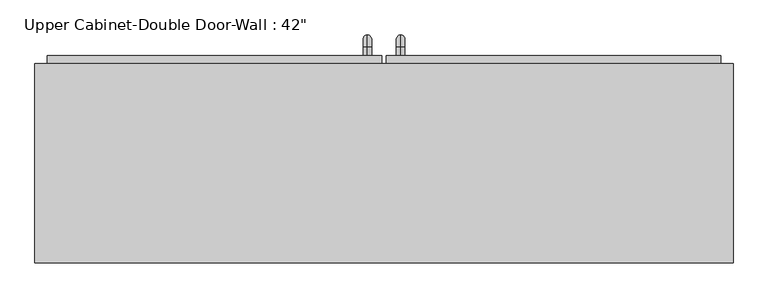
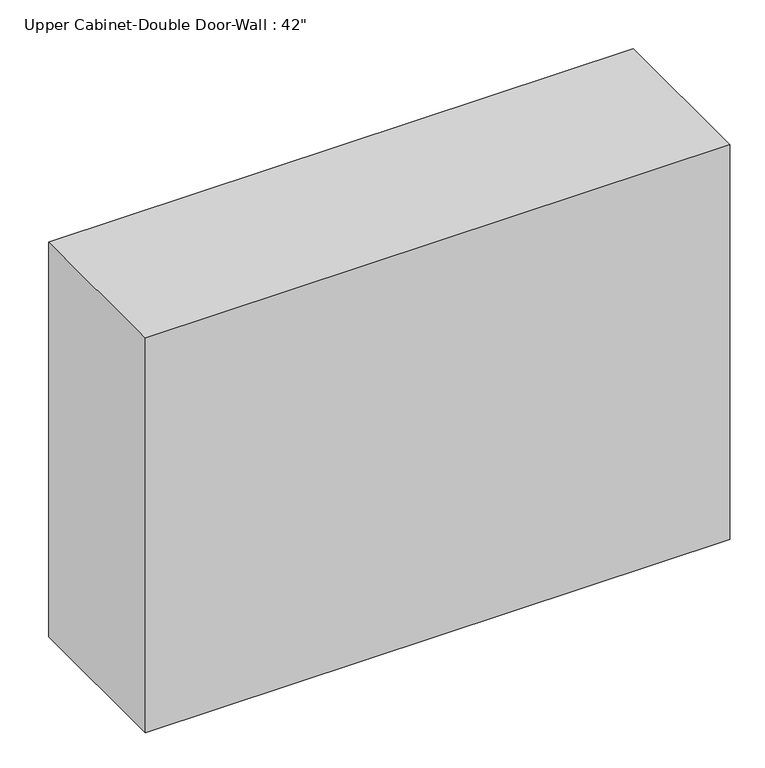
"""IFC4 building model written with IfcOpenShell, lengths in millimetres: furniture geometry."""

import ifcopenshell
import ifcopenshell.guid

model = None  # the IFC model being written
_history = None  # IfcOwnerHistory: only IFC2X3 demands one
_inside = {}  # id of a spatial element -> (the spatial element, [elements in it])
_under = {}  # id of a project, library or spatial element -> (it, [spatial elements below it])
_declared = {}  # id of a project -> (the project, [libraries it declares])
_typed = {}  # id of a type object -> (the type object, [elements of that type])
_made_of = {}  # id of a material, layer set ... -> (it, [elements and type objects made of it])


def new_model(schema):
    """Start an empty IFC model of exactly this schema.

    Asked for "IFC4X3", IfcOpenShell would pick the latest addendum, in which some entities
    have other attributes; the version numbers below select the first issue.
    IFC2X3 requires an IfcOwnerHistory on every rooted entity: one is made here for all.
    """
    global model, _history
    if schema == "IFC4X3":
        model = ifcopenshell.file(schema_version=(4, 3, 0, 0))
    else:
        model = ifcopenshell.file(schema=schema)
    _inside.clear()
    _under.clear()
    _declared.clear()
    _typed.clear()
    _made_of.clear()
    _history = None
    if model.schema == "IFC2X3":
        org = make("IfcOrganization", Name="unknown")
        user = make(
            "IfcPersonAndOrganization",
            ThePerson=make("IfcPerson", FamilyName="unknown"),
            TheOrganization=org,
        )
        app = make(
            "IfcApplication",
            ApplicationDeveloper=org,
            Version="unknown",
            ApplicationFullName="unknown",
            ApplicationIdentifier="unknown",
        )
        _history = make(
            "IfcOwnerHistory",
            OwningUser=user,
            OwningApplication=app,
            ChangeAction="ADDED",
            CreationDate=0,
        )
    return model


def make(cls, **values):
    """One entity of the class cls with the attributes given. An attribute that is None is left unset."""
    return model.create_entity(
        cls, **{name: value for name, value in values.items() if value is not None}
    )


def rooted(cls, **values):
    """An entity with a GlobalId (a new one), such as an element, a storey or a relation."""
    return make(cls, GlobalId=ifcopenshell.guid.new(), OwnerHistory=_history, **values)


def si_unit(unit_type, name, prefix=None):
    """IfcSIUnit, for example si_unit("LENGTHUNIT", "METRE", prefix="MILLI")."""
    return make("IfcSIUnit", UnitType=unit_type, Prefix=prefix, Name=name)


def assignment(units):
    """IfcUnitAssignment: the units of a project."""
    return None if units is None else make("IfcUnitAssignment", Units=units)


def point(xyz):
    """IfcCartesianPoint."""
    return None if xyz is None else make("IfcCartesianPoint", Coordinates=xyz)


def direction(xyz):
    """IfcDirection."""
    return None if xyz is None else make("IfcDirection", DirectionRatios=xyz)


def frame(location, z_axis=None, x_axis=None):
    """IfcAxis2Placement3D, a coordinate frame: its origin and axes. An axis left out is left unset."""
    return make(
        "IfcAxis2Placement3D",
        Location=point(location),
        Axis=direction(z_axis),
        RefDirection=direction(x_axis),
    )


def origin():
    """The frame at (0, 0, 0) with its axes left unset."""
    return frame((0.0, 0.0, 0.0))


def place(relative_to, where):
    """IfcLocalPlacement: puts the frame where relative to a parent placement (None: the world)."""
    return make(
        "IfcLocalPlacement", PlacementRelTo=relative_to, RelativePlacement=where
    )


def context(
    kind, dimensions, precision=None, world=None, true_north=None, identifier=None
):
    """IfcGeometricRepresentationContext, for example the 3D "Model" context."""
    return make(
        "IfcGeometricRepresentationContext",
        ContextIdentifier=identifier,
        ContextType=kind,
        CoordinateSpaceDimension=dimensions,
        Precision=precision,
        WorldCoordinateSystem=world,
        TrueNorth=true_north,
    )


def project(units=None, contexts=None):
    """IfcProject with its units and contexts."""
    return rooted(
        "IfcProject",
        Name="project",
        RepresentationContexts=contexts,
        UnitsInContext=assignment(units),
    )


def spatial(cls, under=None, at=None, **own):
    """A site, building, storey or space (cls), placed at a placement, below another one or the project."""
    s = rooted(cls, ObjectPlacement=at, **own)
    if under is not None:
        _under.setdefault(under.id(), (under, []))[1].append(s)
    return s


def polyline(points):
    """IfcPolyline through the points."""
    return make("IfcPolyline", Points=[point(p) for p in points])


def circle_curve(where, radius):
    """IfcCircle in the frame where."""
    return make("IfcCircle", Position=where, Radius=radius)


def ellipse_curve(where, semi_axis1, semi_axis2):
    """IfcEllipse in the frame where."""
    return make(
        "IfcEllipse", Position=where, SemiAxis1=semi_axis1, SemiAxis2=semi_axis2
    )


def trimmed(basis, trim1, trim2, sense, master):
    """IfcTrimmedCurve: the piece of a basis curve between two trims."""
    return make(
        "IfcTrimmedCurve",
        BasisCurve=basis,
        Trim1=trim1,
        Trim2=trim2,
        SenseAgreement=sense,
        MasterRepresentation=master,
    )


def outline(outer, holes=None, kind="AREA"):
    """IfcArbitraryClosedProfileDef: a profile drawn as a closed curve; with holes, ...WithVoids."""
    if holes is None:
        return make("IfcArbitraryClosedProfileDef", ProfileType=kind, OuterCurve=outer)
    return make(
        "IfcArbitraryProfileDefWithVoids",
        ProfileType=kind,
        OuterCurve=outer,
        InnerCurves=holes,
    )


def extrude(swept, where, along, depth):
    """IfcExtrudedAreaSolid: the profile swept, set in the frame where, extruded along a direction by depth."""
    return make(
        "IfcExtrudedAreaSolid",
        SweptArea=swept,
        Position=where,
        ExtrudedDirection=direction(along),
        Depth=depth,
    )


def faces_of(points, faces, orient=None, outer=None):
    """IfcFace entities. A face is a list of loops; a loop is a list of indices into points, from 0.

    orient and outer hold one flag for each loop. By default every Orientation is true, the
    first loop of a face is its IfcFaceOuterBound and the others are IfcFaceBound.
    """
    made = []
    for i, loops in enumerate(faces):
        bounds = []
        for j, loop in enumerate(loops):
            is_outer = j == 0 if outer is None else outer[i][j]
            bounds.append(
                make(
                    "IfcFaceOuterBound" if is_outer else "IfcFaceBound",
                    Bound=make("IfcPolyLoop", Polygon=[points[k] for k in loop]),
                    Orientation=True if orient is None else orient[i][j],
                )
            )
        made.append(make("IfcFace", Bounds=bounds))
    return made


def faceted_brep(points, faces, orient=None, outer=None, voids=None):
    """IfcFacetedBrep: a solid bounded by flat faces; with voids (closed shells), ...WithVoids."""
    shared = [point(p) for p in points]
    hull = make("IfcClosedShell", CfsFaces=faces_of(shared, faces, orient, outer))
    if voids is None:
        return make("IfcFacetedBrep", Outer=hull)
    return make(
        "IfcFacetedBrepWithVoids",
        Outer=hull,
        Voids=[
            make(cls, CfsFaces=faces_of(shared, fs, o, b)) for cls, fs, o, b in voids
        ],
    )


def shape(context_of_items, identifier, shape_type, items):
    """IfcShapeRepresentation: the items that make up one representation, for example the "Body"."""
    return make(
        "IfcShapeRepresentation",
        ContextOfItems=context_of_items,
        RepresentationIdentifier=identifier,
        RepresentationType=shape_type,
        Items=items,
    )


def source(mapping_origin, context_of_items, identifier, shape_type, items):
    """IfcRepresentationMap: a shape defined once, which mapped items show again and again."""
    return make(
        "IfcRepresentationMap",
        MappingOrigin=mapping_origin,
        MappedRepresentation=shape(context_of_items, identifier, shape_type, items),
    )


def transform(
    local_origin,
    x_axis=None,
    y_axis=None,
    z_axis=None,
    scale=None,
    scale2=None,
    scale3=None,
    uniform=True,
):
    """IfcCartesianTransformationOperator3D, or its non-uniform kind. x_axis, y_axis, z_axis: its Axis1, 2, 3."""
    if uniform:
        return make(
            "IfcCartesianTransformationOperator3D",
            Axis1=direction(x_axis),
            Axis2=direction(y_axis),
            LocalOrigin=point(local_origin),
            Scale=scale,
            Axis3=direction(z_axis),
        )
    return make(
        "IfcCartesianTransformationOperator3DnonUniform",
        Axis1=direction(x_axis),
        Axis2=direction(y_axis),
        LocalOrigin=point(local_origin),
        Scale=scale,
        Axis3=direction(z_axis),
        Scale2=scale2,
        Scale3=scale3,
    )


def mapped(mapping_source, mapping_target):
    """IfcMappedItem: shows the shape of a source again, moved by a transform."""
    return make(
        "IfcMappedItem", MappingSource=mapping_source, MappingTarget=mapping_target
    )


def made_of(thing, what):
    """Note that an element or type object is made of a material, layer set ...; save() writes the relation."""
    if what is not None:
        _made_of.setdefault(what.id(), (what, []))[1].append(thing)
    return thing


def element(
    cls,
    number,
    at=None,
    inside=None,
    cuts=None,
    type_object=None,
    material=None,
    context=None,
    identifier="Body",
    shape_type=None,
    held_by="IfcProductDefinitionShape",
    body=None,
    shapes=None,
    **own,
):
    """One element of the class cls, such as IfcWall. Its Tag is "e" and its number.

    at: its placement. inside: the storey or other place that contains it. cuts: it is an
    opening in that element (IfcRelVoidsElement). A single representation is given by context,
    identifier, shape_type and body (its items); several are given by shapes. held_by: the class
    of the entity that holds the representations. save() writes the other relations.
    """
    e = rooted(cls, Tag="e%d" % number, ObjectPlacement=at, **own)
    if body is not None:
        shapes = [shape(context, identifier, shape_type, body)]
    if shapes is not None:
        e.Representation = make(held_by, Representations=shapes)
    if inside is not None:
        _inside.setdefault(inside.id(), (inside, []))[1].append(e)
    if cuts is not None:
        rooted(
            "IfcRelVoidsElement", RelatingBuildingElement=cuts, RelatedOpeningElement=e
        )
    if type_object is not None:
        _typed.setdefault(type_object.id(), (type_object, []))[1].append(e)
    return made_of(e, material)


def aggregate(whole, parts):
    """IfcRelAggregates: a whole, such as a stair, and the parts it consists of."""
    return rooted("IfcRelAggregates", RelatingObject=whole, RelatedObjects=parts)


def save(model, path):
    """Write the relations noted so far, then the file.

    IfcRelAggregates (storeys below a building ...), IfcRelContainedInSpatialStructure (elements
    in a storey), IfcRelDefinesByType, IfcRelAssociatesMaterial and IfcRelDeclares: one each for
    every whole, place, type object, material and project.
    """
    for whole, parts in _under.values():
        aggregate(whole, parts)
    for where, things in _inside.values():
        rooted(
            "IfcRelContainedInSpatialStructure",
            RelatedElements=things,
            RelatingStructure=where,
        )
    for kind, things in _typed.values():
        rooted("IfcRelDefinesByType", RelatedObjects=things, RelatingType=kind)
    for what, things in _made_of.values():
        rooted("IfcRelAssociatesMaterial", RelatedObjects=things, RelatingMaterial=what)
    for by, libraries in _declared.values():
        rooted("IfcRelDeclares", RelatingContext=by, RelatedDefinitions=libraries)
    model.write(path)


def plane_surface(at):
    """IfcPlane: the flat surface through the origin of the frame at, square to its z axis."""
    return make("IfcPlane", Position=at)


def cylinder_surface(at, radius):
    """IfcCylindricalSurface: all points at the distance radius from the z axis of the frame at."""
    return make("IfcCylindricalSurface", Position=at, Radius=radius)


def revolved_surface(curve, axis_point, axis_direction):
    """IfcSurfaceOfRevolution: the curve turned about the line through axis_point along axis_direction."""
    return make(
        "IfcSurfaceOfRevolution",
        SweptCurve=make("IfcArbitraryOpenProfileDef", ProfileType="CURVE", Curve=curve),
        AxisPosition=make("IfcAxis1Placement", Location=point(axis_point), Axis=direction(axis_direction)),
    )


def advanced_brep(points, edges, surfaces, faces):
    """IfcAdvancedBrep: a solid bounded by faces that lie on surfaces and meet in shared edges.

    An edge is (start, end): straight between two places in points (the first is 0);
    or (start, end, curve); or (start, end, curve, False) where it runs against its curve.
    A face is (place in surfaces, loops), or (place, loops, False) where it looks against
    its surface's normal. A loop lists edges by number (the first is 1), with a minus sign
    where the edge is run from its end to its start. The first loop is the outer one.
    """
    corners = [point(p) for p in points]
    vertices = [make("IfcVertexPoint", VertexGeometry=c) for c in corners]
    made = []
    for start, end, *more in edges:
        made.append(
            make(
                "IfcEdgeCurve",
                EdgeStart=vertices[start],
                EdgeEnd=vertices[end],
                EdgeGeometry=more[0] if more else make("IfcPolyline", Points=[corners[start], corners[end]]),
                SameSense=more[1] if len(more) > 1 else True,
            )
        )
    hull = []
    for where, loops, *sense in faces:
        bounds = []
        for j, loop in enumerate(loops):
            ring = [make("IfcOrientedEdge", EdgeElement=made[abs(k) - 1], Orientation=k > 0) for k in loop]
            bounds.append(
                make(
                    "IfcFaceOuterBound" if j == 0 else "IfcFaceBound",
                    Bound=make("IfcEdgeLoop", EdgeList=ring),
                    Orientation=True,
                )
            )
        hull.append(make("IfcAdvancedFace", Bounds=bounds, FaceSurface=surfaces[where], SameSense=sense[0] if sense else True))
    return make("IfcAdvancedBrep", Outer=make("IfcClosedShell", CfsFaces=hull))


def furniture_35403546(model_context):
    return source(origin(), model_context, "Body", "SolidModel", [
        faceted_brep([(-503.6288372, 61.9125, 2133.6), (-503.6288372, 61.9125, 1371.6), (563.1711628, 61.9125, 1371.6), (563.1711628, 61.9125, 2133.6), (-503.6288372, 366.7125, 2133.6), (563.1711628, 366.7125, 2133.6), (563.1711628, 366.7125, 1371.6), (-503.6288372, 366.7125, 1371.6), (-484.5788372, 366.7125, 2114.55), (-484.5788372, 366.7125, 1390.65), (544.1211628, 366.7125, 1390.65), (544.1211628, 366.7125, 2114.55), (544.1211628, 80.9625, 2114.55), (-484.5788372, 80.9625, 2114.55), (544.1211628, 80.9625, 1390.65), (-484.5788372, 80.9625, 1390.65)], [[[0, 1, 2, 3]], [[4, 5, 6, 7], [8, 9, 10, 11]], [[1, 0, 4, 7]], [[2, 1, 7, 6]], [[3, 2, 6, 5]], [[0, 3, 5, 4]], [[8, 11, 12, 13]], [[11, 10, 14, 12]], [[10, 9, 15, 14]], [[9, 8, 13, 15]], [[13, 12, 14, 15]]]),
        advanced_brep(
        [(55.1711628, 379.4125, 1517.65), (55.1711628, 379.4125, 1530.35), (55.1711628, 392.1125, 1517.65), (55.1711628, 392.1125, 1530.35), (55.1711628, 411.1625, 1511.3), (55.1711628, 398.4625, 1511.3), (55.1711628, 398.4625, 1435.1), (55.1711628, 411.1625, 1435.1), (55.1711628, 392.1125, 1416.05), (55.1711628, 392.1125, 1428.75), (55.1711628, 379.4125, 1428.75), (55.1711628, 379.4125, 1416.05)],
        [
            (0, 1, circle_curve(frame((55.1711628, 379.4125, 1524.0), z_axis=(0.0, -1.0, 0.0), x_axis=(0.0, 0.0, -1.0)), 6.35)),
            (1, 0, circle_curve(frame((55.1711628, 379.4125, 1524.0), z_axis=(0.0, -1.0, 0.0), x_axis=(0.0, 0.0, -1.0)), 6.35)),
            (0, 2),
            (2, 3, circle_curve(frame((55.1711628, 392.1125, 1524.0), z_axis=(0.0, -1.0, 0.0), x_axis=(0.0, 0.0, -1.0)), 6.35)),
            (3, 1),
            (3, 2, circle_curve(frame((55.1711628, 392.1125, 1524.0), z_axis=(0.0, -1.0, 0.0), x_axis=(0.0, 0.0, -1.0)), 6.35)),
            (4, 3, circle_curve(frame((55.1711628, 392.1125, 1511.3), z_axis=(1.0, 0.0, 0.0), x_axis=(0.0, 0.0, 1.0)), 19.05)),
            (2, 5, circle_curve(frame((55.1711628, 392.1125, 1511.3), z_axis=(-1.0, 0.0, 0.0), x_axis=(0.0, 0.0, 1.0)), 6.35)),
            (5, 4, circle_curve(frame((55.1711628, 404.8125, 1511.3), z_axis=(0.0, 0.0, 1.0), x_axis=(0.0, -1.0, 0.0)), 6.35)),
            (4, 5, circle_curve(frame((55.1711628, 404.8125, 1511.3), z_axis=(0.0, 0.0, 1.0), x_axis=(0.0, -1.0, 0.0)), 6.35)),
            (5, 6),
            (6, 7, circle_curve(frame((55.1711628, 404.8125, 1435.1), z_axis=(0.0, 0.0, 1.0), x_axis=(0.0, -1.0, 0.0)), 6.35)),
            (7, 4),
            (7, 6, circle_curve(frame((55.1711628, 404.8125, 1435.1), z_axis=(0.0, 0.0, 1.0), x_axis=(0.0, -1.0, 0.0)), 6.35)),
            (8, 7, circle_curve(frame((55.1711628, 392.1125, 1435.1), z_axis=(1.0, 0.0, 0.0), x_axis=(0.0, 1.0, 0.0)), 19.05)),
            (6, 9, circle_curve(frame((55.1711628, 392.1125, 1435.1), z_axis=(-1.0, 0.0, 0.0), x_axis=(0.0, 1.0, 0.0)), 6.35)),
            (9, 8, circle_curve(frame((55.1711628, 392.1125, 1422.4), z_axis=(0.0, 1.0, 0.0), x_axis=(0.0, 0.0, 1.0)), 6.35)),
            (8, 9, circle_curve(frame((55.1711628, 392.1125, 1422.4), z_axis=(0.0, 1.0, 0.0), x_axis=(0.0, 0.0, 1.0)), 6.35)),
            (10, 11, circle_curve(frame((55.1711628, 379.4125, 1422.4), z_axis=(0.0, -1.0, 0.0), x_axis=(0.0, 0.0, 1.0)), 6.35)),
            (11, 10, circle_curve(frame((55.1711628, 379.4125, 1422.4), z_axis=(0.0, -1.0, 0.0), x_axis=(0.0, 0.0, 1.0)), 6.35)),
            (9, 10),
            (11, 8),
        ],
        [
            plane_surface(frame((48.8211628, 379.4125, 1524.0), z_axis=(0.0, -1.0, 0.0), x_axis=(0.0, 0.0, 1.0))),
            cylinder_surface(frame((55.1711628, 379.4125, 1524.0), z_axis=(0.0, -1.0, 0.0), x_axis=(0.0, 0.0, -1.0)), 6.35),
            revolved_surface(trimmed(ellipse_curve(frame((55.1711628, 392.1125, 1524.0), z_axis=(0.0, -1.0, 0.0), x_axis=(0.0, 0.0, -1.0)), 6.35, 6.35), [point((55.1711628, 392.1125, 1517.65))], [point((55.1711628, 392.1125, 1530.35))], True, "CARTESIAN"), (55.1711628, 392.1125, 1511.3), (-1.0, 0.0, 0.0)),
            revolved_surface(trimmed(ellipse_curve(frame((55.1711628, 392.1125, 1524.0), z_axis=(0.0, -1.0, 0.0), x_axis=(0.0, 0.0, -1.0)), 6.35, 6.35), [point((55.1711628, 392.1125, 1530.35))], [point((55.1711628, 392.1125, 1517.65))], True, "CARTESIAN"), (55.1711628, 392.1125, 1511.3), (-1.0, 0.0, 0.0)),
            cylinder_surface(frame((55.1711628, 404.8125, 1511.3), z_axis=(0.0, 0.0, 1.0), x_axis=(0.0, -1.0, 0.0)), 6.35),
            revolved_surface(trimmed(ellipse_curve(frame((55.1711628, 404.8125, 1435.1), z_axis=(0.0, 0.0, 1.0), x_axis=(0.0, -1.0, 0.0)), 6.35, 6.35), [point((55.1711628, 398.4625, 1435.1))], [point((55.1711628, 411.1625, 1435.1))], True, "CARTESIAN"), (55.1711628, 392.1125, 1435.1), (-1.0, 0.0, 0.0)),
            revolved_surface(trimmed(ellipse_curve(frame((55.1711628, 404.8125, 1435.1), z_axis=(0.0, 0.0, 1.0), x_axis=(0.0, -1.0, 0.0)), 6.35, 6.35), [point((55.1711628, 411.1625, 1435.1))], [point((55.1711628, 398.4625, 1435.1))], True, "CARTESIAN"), (55.1711628, 392.1125, 1435.1), (-1.0, 0.0, 0.0)),
            plane_surface(frame((48.8211628, 379.4125, 1422.4), z_axis=(0.0, -1.0, 0.0), x_axis=(0.0, 0.0, -1.0))),
            cylinder_surface(frame((55.1711628, 392.1125, 1422.4), z_axis=(0.0, 1.0, 0.0), x_axis=(0.0, 0.0, 1.0)), 6.35),
        ],
        [
            (0, [[1, 2]]),
            (1, [[-1, 3, 4, 5]]),
            (1, [[-2, -5, 6, -3]]),
            (2, [[7, -4, 8, 9]]),
            (3, [[-8, -6, -7, 10]]),
            (4, [[-9, 11, 12, 13]]),
            (4, [[-10, -13, 14, -11]]),
            (5, [[15, -12, 16, 17]]),
            (6, [[-16, -14, -15, 18]]),
            (7, [[19, 20]]),
            (8, [[-17, 21, -20, 22]]),
            (8, [[-18, -22, -19, -21]]),
        ],
    ),
        advanced_brep(
        [(4.3711628, 379.4125, 1517.65), (4.3711628, 379.4125, 1530.35), (4.3711628, 392.1125, 1517.65), (4.3711628, 392.1125, 1530.35), (4.3711628, 411.1625, 1511.3), (4.3711628, 398.4625, 1511.3), (4.3711628, 398.4625, 1435.1), (4.3711628, 411.1625, 1435.1), (4.3711628, 392.1125, 1416.05), (4.3711628, 392.1125, 1428.75), (4.3711628, 379.4125, 1428.75), (4.3711628, 379.4125, 1416.05)],
        [
            (0, 1, circle_curve(frame((4.3711628, 379.4125, 1524.0), z_axis=(0.0, -1.0, 0.0), x_axis=(0.0, 0.0, 1.0)), 6.35)),
            (1, 0, circle_curve(frame((4.3711628, 379.4125, 1524.0), z_axis=(0.0, -1.0, 0.0), x_axis=(0.0, 0.0, 1.0)), 6.35)),
            (0, 2),
            (2, 3, circle_curve(frame((4.3711628, 392.1125, 1524.0), z_axis=(0.0, -1.0, 0.0), x_axis=(0.0, 0.0, 1.0)), 6.35)),
            (3, 1),
            (3, 2, circle_curve(frame((4.3711628, 392.1125, 1524.0), z_axis=(0.0, -1.0, 0.0), x_axis=(0.0, 0.0, 1.0)), 6.35)),
            (4, 3, circle_curve(frame((4.3711628, 392.1125, 1511.3), z_axis=(1.0, 0.0, 0.0), x_axis=(0.0, 0.0, 1.0)), 19.05)),
            (2, 5, circle_curve(frame((4.3711628, 392.1125, 1511.3), z_axis=(-1.0, 0.0, 0.0), x_axis=(0.0, 0.0, 1.0)), 6.35)),
            (5, 4, circle_curve(frame((4.3711628, 404.8125, 1511.3), z_axis=(0.0, 0.0, 1.0), x_axis=(0.0, 1.0, 0.0)), 6.35)),
            (4, 5, circle_curve(frame((4.3711628, 404.8125, 1511.3), z_axis=(0.0, 0.0, 1.0), x_axis=(0.0, 1.0, 0.0)), 6.35)),
            (5, 6),
            (6, 7, circle_curve(frame((4.3711628, 404.8125, 1435.1), z_axis=(0.0, 0.0, 1.0), x_axis=(0.0, 1.0, 0.0)), 6.35)),
            (7, 4),
            (7, 6, circle_curve(frame((4.3711628, 404.8125, 1435.1), z_axis=(0.0, 0.0, 1.0), x_axis=(0.0, 1.0, 0.0)), 6.35)),
            (8, 7, circle_curve(frame((4.3711628, 392.1125, 1435.1), z_axis=(1.0, 0.0, 0.0), x_axis=(0.0, 1.0, 0.0)), 19.05)),
            (6, 9, circle_curve(frame((4.3711628, 392.1125, 1435.1), z_axis=(-1.0, 0.0, 0.0), x_axis=(0.0, 1.0, 0.0)), 6.35)),
            (9, 8, circle_curve(frame((4.3711628, 392.1125, 1422.4), z_axis=(0.0, 1.0, 0.0), x_axis=(0.0, 0.0, -1.0)), 6.35)),
            (8, 9, circle_curve(frame((4.3711628, 392.1125, 1422.4), z_axis=(0.0, 1.0, 0.0), x_axis=(0.0, 0.0, -1.0)), 6.35)),
            (10, 11, circle_curve(frame((4.3711628, 379.4125, 1422.4), z_axis=(0.0, -1.0, 0.0), x_axis=(0.0, 0.0, -1.0)), 6.35)),
            (11, 10, circle_curve(frame((4.3711628, 379.4125, 1422.4), z_axis=(0.0, -1.0, 0.0), x_axis=(0.0, 0.0, -1.0)), 6.35)),
            (9, 10),
            (11, 8),
        ],
        [
            plane_surface(frame((-1.9788372, 379.4125, 1524.0), z_axis=(0.0, -1.0, 0.0), x_axis=(0.0, 0.0, 1.0))),
            cylinder_surface(frame((4.3711628, 379.4125, 1524.0), z_axis=(0.0, -1.0, 0.0), x_axis=(0.0, 0.0, 1.0)), 6.35),
            revolved_surface(trimmed(ellipse_curve(frame((4.3711628, 392.1125, 1524.0), z_axis=(0.0, -1.0, 0.0), x_axis=(0.0, 0.0, 1.0)), 6.35, 6.35), [point((4.3711628, 392.1125, 1517.65))], [point((4.3711628, 392.1125, 1530.35))], True, "CARTESIAN"), (4.3711628, 392.1125, 1511.3), (-1.0, 0.0, 0.0)),
            revolved_surface(trimmed(ellipse_curve(frame((4.3711628, 392.1125, 1524.0), z_axis=(0.0, -1.0, 0.0), x_axis=(0.0, 0.0, 1.0)), 6.35, 6.35), [point((4.3711628, 392.1125, 1530.35))], [point((4.3711628, 392.1125, 1517.65))], True, "CARTESIAN"), (4.3711628, 392.1125, 1511.3), (-1.0, 0.0, 0.0)),
            cylinder_surface(frame((4.3711628, 404.8125, 1511.3), z_axis=(0.0, 0.0, 1.0), x_axis=(0.0, 1.0, 0.0)), 6.35),
            revolved_surface(trimmed(ellipse_curve(frame((4.3711628, 404.8125, 1435.1), z_axis=(0.0, 0.0, 1.0), x_axis=(0.0, 1.0, 0.0)), 6.35, 6.35), [point((4.3711628, 398.4625, 1435.1))], [point((4.3711628, 411.1625, 1435.1))], True, "CARTESIAN"), (4.3711628, 392.1125, 1435.1), (-1.0, 0.0, 0.0)),
            revolved_surface(trimmed(ellipse_curve(frame((4.3711628, 404.8125, 1435.1), z_axis=(0.0, 0.0, 1.0), x_axis=(0.0, 1.0, 0.0)), 6.35, 6.35), [point((4.3711628, 411.1625, 1435.1))], [point((4.3711628, 398.4625, 1435.1))], True, "CARTESIAN"), (4.3711628, 392.1125, 1435.1), (-1.0, 0.0, 0.0)),
            plane_surface(frame((-1.9788372, 379.4125, 1422.4), z_axis=(0.0, -1.0, 0.0), x_axis=(0.0, 0.0, -1.0))),
            cylinder_surface(frame((4.3711628, 392.1125, 1422.4), z_axis=(0.0, 1.0, 0.0), x_axis=(0.0, 0.0, -1.0)), 6.35),
        ],
        [
            (0, [[1, 2]]),
            (1, [[-1, 3, 4, 5]]),
            (1, [[-2, -5, 6, -3]]),
            (2, [[7, -4, 8, 9]]),
            (3, [[-8, -6, -7, 10]]),
            (4, [[-9, 11, 12, 13]]),
            (4, [[-10, -13, 14, -11]]),
            (5, [[15, -12, 16, 17]]),
            (6, [[-16, -14, -15, 18]]),
            (7, [[19, 20]]),
            (8, [[-17, 21, -20, 22]]),
            (8, [[-18, -22, -19, -21]]),
        ],
    ),
        extrude(outline(polyline([(32.9461628, 379.4125), (544.1211628, 379.4125), (544.1211628, 347.6625), (32.9461628, 347.6625), (32.9461628, 379.4125)])), frame((0.0, 0.0, 1390.65), z_axis=(0.0, 0.0, 1.0), x_axis=(1.0, 0.0, 0.0)), (0.0, 0.0, 1.0), 723.9),
        extrude(outline(polyline([(-484.5788372, 379.4125), (26.5961628, 379.4125), (26.5961628, 347.6625), (-484.5788372, 347.6625), (-484.5788372, 379.4125)])), frame((0.0, 0.0, 1390.65), z_axis=(0.0, 0.0, 1.0), x_axis=(1.0, 0.0, 0.0)), (0.0, 0.0, 1.0), 723.9),
    ])


if __name__ == "__main__":
    model = new_model("IFC4")
    model_context = context("Model", 3, world=origin())
    ifc_project = project(units=[si_unit("LENGTHUNIT", "METRE", prefix="MILLI")], contexts=[model_context])
    site = spatial("IfcSite", under=ifc_project)
    building = spatial("IfcBuilding", under=site)
    placement = place(None, origin())
    furniture_shape = furniture_35403546(model_context)
    element("IfcFurniture", 1, ObjectType="Upper Cabinet-Double Door-Wall : 42\"", at=placement, inside=building, context=model_context, shape_type="MappedRepresentation", body=[
        mapped(furniture_shape, transform((0.0, 0.0, 0.0), x_axis=(1.0, 0.0, 0.0), y_axis=(0.0, 1.0, 0.0), z_axis=(0.0, 0.0, 1.0))),
    ])
    save(model, "model.ifc")

# Revit data of these elements
# Type "Upper Cabinet-Double Door-Wall : 42\""
#   Assembly Code = "C1030410"
#   Depth = 1' - 0"
#   Height = 2' - 6"
#   Top Of Cabinet = 7' - 0"
#   Width = 3' - 6"
#   Cabinet Material = none
#   Door/Drawer Material = none
#   Handle Material = Cabinets - Handles
#   Default Elevation = 0
# Element 1 (IfcFurniture, "Upper Cabinet-Double Door-Wall : 42\"")
#   Materials on its faces: "Cabinets - Handles", "Cabinets"
# Materials
#   "Cabinets - Handles": class "Metal", colour RGB 57 57 57, transparency 0
#   "Cabinets": class "Miscellaneous", colour RGB 249 249 249, transparency 0
